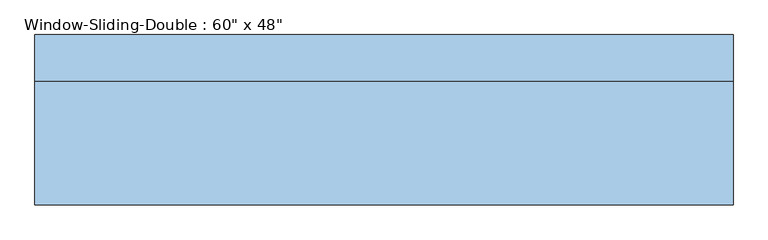
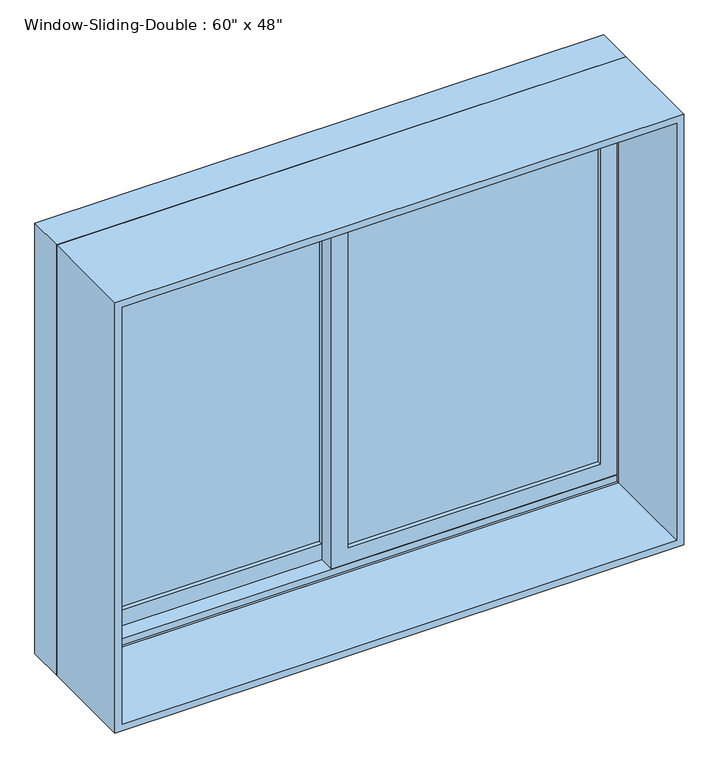
"""IFC4 building model written with IfcOpenShell, lengths in millimetres: window geometry."""

from ifc_helpers import new_model, si_unit, frame, origin, place, context, project, spatial, polyline, outline, extrude, faceted_brep, source, transform, mapped, element, save


def window_0d2bb1db(model_context):
    return source(origin(), model_context, "Body", "SolidModel", [
        faceted_brep([(-762.0, 89.8525, 914.4), (-762.0, 191.4525, 914.4), (762.0, 191.4525, 914.4), (762.0, 89.8525, 914.4), (-721.0778905, 191.4525, 2092.6778905), (-721.0778905, 185.1025, 2092.6778905), (-721.0778905, 185.1025, 933.45), (-721.0778905, 191.4525, 933.45), (721.0778905, 185.1025, 2092.6778905), (721.0778905, 185.1025, 933.45), (742.95, 185.1025, 933.45), (742.95, 185.1025, 2114.55), (-742.95, 185.1025, 2114.55), (-742.95, 185.1025, 933.45), (-742.95, 89.8525, 2114.55), (-742.95, 89.8525, 933.45), (-742.95, 96.2025, 933.45), (-742.95, 96.2025, 952.5), (-742.95, 140.6525, 952.5), (-742.95, 140.6525, 933.45), (762.0, 89.8525, 2133.6), (-762.0, 89.8525, 2133.6), (742.95, 89.8525, 2114.55), (742.95, 89.8525, 933.45), (-762.0, 191.4525, 2133.6), (762.0, 191.4525, 2133.6), (721.0778905, 191.4525, 933.45), (721.0778905, 191.4525, 2092.6778905), (742.95, 140.6525, 933.45), (742.95, 140.6525, 952.5), (742.95, 96.2025, 952.5), (742.95, 96.2025, 933.45)], [[[0, 1, 2, 3]], [[4, 5, 6, 7]], [[5, 8, 9, 10, 11, 12, 13, 6]], [[12, 14, 15, 16, 17, 18, 19, 13]], [[0, 3, 20, 21], [22, 23, 15, 14]], [[24, 1, 0, 21]], [[2, 1, 24, 25], [4, 7, 26, 27]], [[5, 4, 27, 8]], [[12, 11, 22, 14]], [[21, 20, 25, 24]], [[8, 27, 26, 9]], [[22, 11, 10, 28, 29, 30, 31, 23]], [[20, 3, 2, 25]], [[26, 7, 6, 13, 19, 28, 10, 9]], [[28, 19, 18, 29]], [[29, 18, 17, 30]], [[30, 17, 16, 31]], [[15, 23, 31, 16]]]),
        extrude(outline(polyline([(2133.6, -762.0), (914.4, -762.0), (914.4, 762.0), (2133.6, 762.0), (2133.6, -762.0)]), holes=[polyline([(2114.55, 742.95), (933.45, 742.95), (933.45, -742.95), (2114.55, -742.95), (2114.55, 742.95)])]), frame((0.0, -180.0225, 0.0), z_axis=(0.0, 1.0, 0.0), x_axis=(0.0, 0.0, 1.0)), (0.0, 0.0, 1.0), 269.875),
        extrude(outline(polyline([(698.5, 127.9525), (698.5, 121.6025), (22.225, 121.6025), (22.225, 127.9525), (698.5, 127.9525)])), frame((0.0, 0.0, 996.95), z_axis=(0.0, 0.0, 1.0), x_axis=(1.0, 0.0, 0.0)), (0.0, 0.0, 1.0), 1073.15),
        extrude(outline(polyline([(698.5, 115.2525), (698.5, 108.9025), (22.225, 108.9025), (22.225, 115.2525), (698.5, 115.2525)])), frame((0.0, 0.0, 996.95), z_axis=(0.0, 0.0, 1.0), x_axis=(1.0, 0.0, 0.0)), (0.0, 0.0, 1.0), 1073.15),
        extrude(outline(polyline([(-22.225, 172.4025), (-22.225, 166.0525), (-698.5, 166.0525), (-698.5, 172.4025), (-22.225, 172.4025)])), frame((0.0, 0.0, 996.95), z_axis=(0.0, 0.0, 1.0), x_axis=(1.0, 0.0, 0.0)), (0.0, 0.0, 1.0), 1073.15),
        extrude(outline(polyline([(-22.225, 159.7025), (-22.225, 153.3525), (-698.5, 153.3525), (-698.5, 159.7025), (-22.225, 159.7025)])), frame((0.0, 0.0, 996.95), z_axis=(0.0, 0.0, 1.0), x_axis=(1.0, 0.0, 0.0)), (0.0, 0.0, 1.0), 1073.15),
        extrude(outline(polyline([(933.45, -742.95), (933.45, 22.225), (2114.55, 22.225), (2114.55, -742.95), (933.45, -742.95)]), holes=[polyline([(2070.1, -22.225), (996.95, -22.225), (996.95, -698.5), (2070.1, -698.5), (2070.1, -22.225)])]), frame((0.0, 140.6525, 0.0), z_axis=(0.0, 1.0, 0.0), x_axis=(0.0, 0.0, 1.0)), (0.0, 0.0, 1.0), 44.45),
        extrude(outline(polyline([(952.5, 742.95), (2114.55, 742.95), (2114.55, -22.225), (952.5, -22.225), (952.5, 742.95)]), holes=[polyline([(996.95, 22.225), (2070.1, 22.225), (2070.1, 698.5), (996.95, 698.5), (996.95, 22.225)])]), frame((0.0, 96.2025, 0.0), z_axis=(0.0, 1.0, 0.0), x_axis=(0.0, 0.0, 1.0)), (0.0, 0.0, 1.0), 44.45),
    ])


if __name__ == "__main__":
    model = new_model("IFC4")
    model_context = context("Model", 3, world=origin())
    ifc_project = project(units=[si_unit("LENGTHUNIT", "METRE", prefix="MILLI")], contexts=[model_context])
    site = spatial("IfcSite", under=ifc_project)
    building = spatial("IfcBuilding", under=site)
    placement = place(None, origin())
    window_shape = window_0d2bb1db(model_context)
    element("IfcWindow", 1, ObjectType="Window-Sliding-Double : 60\" x 48\"", at=placement, inside=building, context=model_context, shape_type="MappedRepresentation", body=[
        mapped(window_shape, transform((0.0, 0.0, 0.0), x_axis=(1.0, 0.0, 0.0), y_axis=(0.0, 1.0, 0.0), z_axis=(0.0, 0.0, 1.0))),
    ])
    save(model, "model.ifc")

# Revit data of these elements
# Type "Window-Sliding-Double : 60\" x 48\""
#   Type Mark = "13"
#   Fire Rating = "0.5h"
#   Assembly Code = "B2020100"
#   Analytic Construction = "Double glazing - domestic"
#   Window Inset [instance default] = 0' - 0"
#   Wall Thickness [instance default] = 0' - 6"
#   Visual Light Transmittance = 0.81
#   Thermal Resistance (R) = 1.8146 (h·ft²·°F)/BTU
#   Solar Heat Gain Coefficient = 0.76
#   Muntin Width = 2' - 2 5/8"
#   Muntin Height = 3' - 6 1/4"
#   Interior Wall Closure [instance default] = 0' - 2 3/4"
#   Heat Transfer Coefficient (U) = 0.5511 BTU/(h·ft²·°F)
#   Frame Extension [instance default] = 0' - 0 1/4"
#   Exterior Wall Closure [instance default] = 0' - 1 1/4"
#   Rough Width = 5' - 0 1/2"
#   Rough Height = 4' - 0 1/2"
#   Height = 4' - 0"
#   Extension Jamb [instance default] = 0' - 2 3/4"
#   Default Sill Height = 3' - 0"
#   Width = 5' - 0"
#   Interior Trim Visibility [instance default] = yes
#   Indicator Visibility [instance default] = yes
#   Exterior Trim Visibility [instance default] = yes
#   Muntin Visibility = yes
#   Extension Jamb Visibility [instance default] = yes
#   Define Thermal Properties by = 1
#   Muntin Pattern = Muntin Pattern_2x2 : Muntin Pattern_2x2
#   Interior Trim Material = Cherry
#   Interior Trim = Trim-Window-Interior-Flat : Picture Frame
#   Interior Frame Material = Cherry
#   Glass Panel Material = Glass, Clear Glazing
#   Exterior Trim Material = PVC, Flexible
#   Exterior Trim = Trim-Window-Exterior-Flat : with Sill
#   Exterior Frame Material = PVC, Flexible
#   Wall Closure = (empty or 0)
# Element 1 (IfcWindow, "Window-Sliding-Double : 60\" x 48\"")
#   Wall Thickness = 1' - 1 7/8"
#   Extension Jamb = 0' - 10 5/8"
#   Materials on its faces: "Cherry", "Glass, Clear Glazing", "PVC, Flexible"
# Materials
#   "Cherry": class "Wood", colour RGB 157 77 38, transparency 0, Description = "Prunus Serotina", Cost = 0
#   "Glass, Clear Glazing": class "Glass", colour RGB 120 120 120, transparency 0, Description = "Clear glazing", Cost = 0
#   "PVC, Flexible": class "Plastic", colour RGB 178 178 178, transparency 0, Description = "Flexible polyvinyl chloride", Cost = 0
